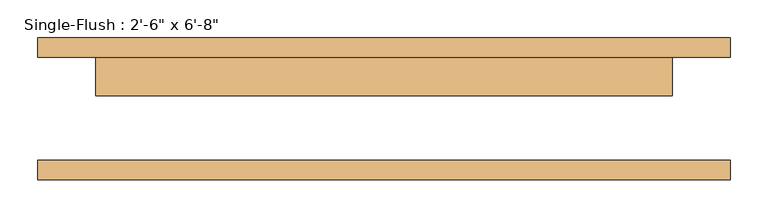
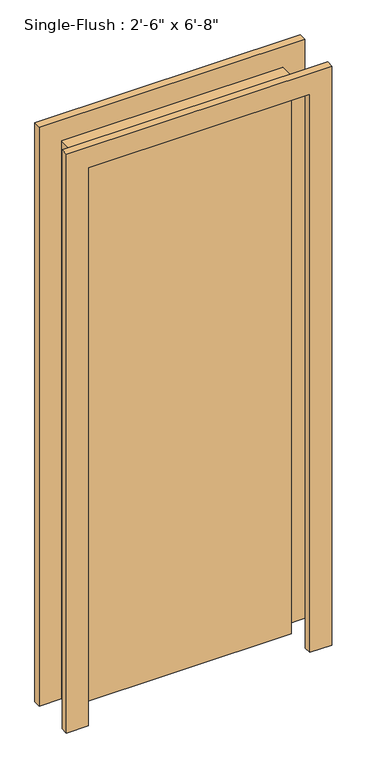
"""IFC4 building model written with IfcOpenShell, lengths in millimetres: door geometry."""

from ifc_helpers import new_model, si_unit, frame, origin, origin_with_axes, place, context, project, spatial, polyline, outline, extrude, source, transform, mapped, element, save


def door_0b154108(model_context):
    return source(origin(), model_context, "Body", "SweptSolid", [
        extrude(outline(polyline([(2108.2, -457.2), (0.0, -457.2), (0.0, -381.0), (2032.0, -381.0), (2032.0, 381.0), (0.0, 381.0), (0.0, 457.2), (2108.2, 457.2), (2108.2, -457.2)])), frame((0.0, 68.2625, 0.0), z_axis=(0.0, 1.0, 0.0), x_axis=(0.0, 0.0, 1.0)), (0.0, 0.0, 1.0), 25.4),
        extrude(outline(polyline([(2108.2, 457.2), (2108.2, -457.2), (0.0, -457.2), (0.0, -381.0), (2032.0, -381.0), (2032.0, 381.0), (0.0, 381.0), (0.0, 457.2), (2108.2, 457.2)])), frame((0.0, -93.6625, 0.0), z_axis=(0.0, 1.0, 0.0), x_axis=(0.0, 0.0, 1.0)), (0.0, 0.0, 1.0), 25.4),
        extrude(outline(polyline([(381.0, 17.4625), (-381.0, 17.4625), (-381.0, 68.2625), (381.0, 68.2625), (381.0, 17.4625)])), origin_with_axes(), (0.0, 0.0, 1.0), 2032.0),
    ])


if __name__ == "__main__":
    model = new_model("IFC4")
    model_context = context("Model", 3, world=origin())
    ifc_project = project(units=[si_unit("LENGTHUNIT", "METRE", prefix="MILLI")], contexts=[model_context])
    site = spatial("IfcSite", under=ifc_project)
    building = spatial("IfcBuilding", under=site)
    placement = place(None, origin())
    door_shape = door_0b154108(model_context)
    element("IfcDoor", 1, ObjectType="Single-Flush : 2'-6\" x 6'-8\"", at=placement, inside=building, context=model_context, shape_type="MappedRepresentation", body=[
        mapped(door_shape, transform((0.0, 0.0, 0.0), x_axis=(1.0, 0.0, 0.0), y_axis=(0.0, 1.0, 0.0), z_axis=(0.0, 0.0, 1.0))),
    ])
    save(model, "model.ifc")

# Revit data of these elements
# Project information
#   Project Issue Date = "Issue Date"
#   Project Status = "Project Status"
#   Client Name = "Owner"
#   Project Address = "Enter address here"
#   Project Name = "Project Name"
#   Project Number = "Project Number"
# Type "Single-Flush : 2'-6\" x 6'-8\""
#   Type Mark = "13"
#   Construction Type Id = "MDOOR"
#   Assembly Code = "C1020"
#   Analytic Construction = "Metal"
#   Thickness = 0' - 2"
#   Heat Transfer Coefficient (U) = 3.7021 W/(m²·K)
#   Height = 6' - 8"
#   Trim Projection Ext = 0' - 1"
#   Trim Projection Int = 0' - 1"
#   Trim Width = 0' - 3"
#   Width = 2' - 6"
#   Door Material = Door - Panel
#   Frame Material = Door - Frame
#   Visual Light Transmittance = 0
#   Solar Heat Gain Coefficient = 0
#   Function = (empty or 0)
#   Wall Closure = (empty or 0)
# Element 1 (IfcDoor, "Single-Flush : 2'-6\" x 6'-8\"")
#   Materials on its faces: "Door - Frame", "Door - Panel"
# Materials
#   "Door - Panel": class "Wood", colour RGB 210 159 95, transparency 0, Cost = 0
#   "Door - Frame": class "Miscellaneous", colour RGB 118 70 51, transparency 0, Cost = 0
